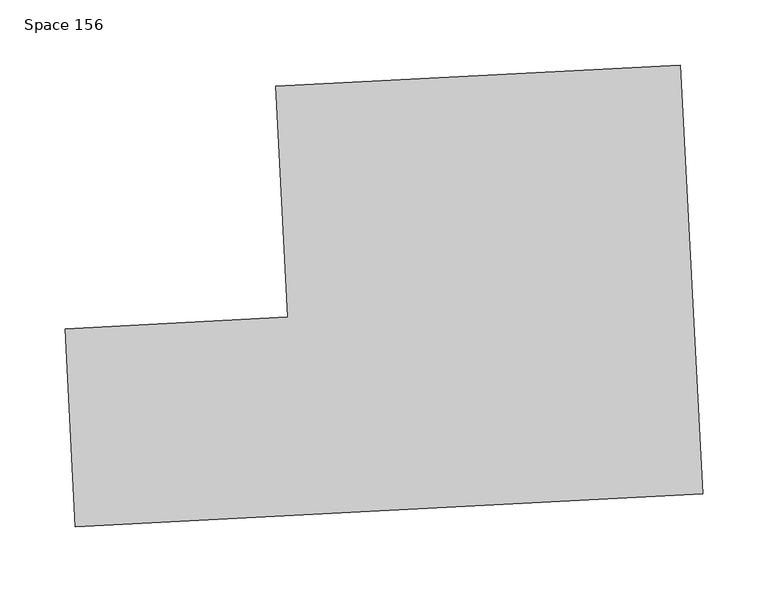
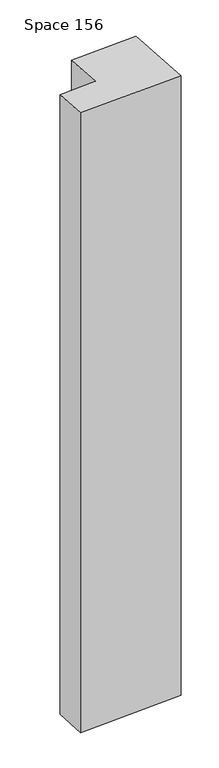
"""IFC4 building model written with IfcOpenShell, lengths in millimetres: proxy geometry, Space 156."""

from ifc_helpers import new_model, si_unit, frame, origin, place, context, project, spatial, polyline, outline, extrude, source, transform, mapped, element, save


def space_156_bf02bf6d(model_context):
    return source(origin(), model_context, "Body", "SweptSolid", [
        extrude(outline(polyline([(6675.6990245, -35006.9418992), (6667.7230248, -34854.7507581), (6838.9380585, -34845.7777585), (6829.6327255, -34668.2214272), (7140.3563053, -34651.9370944), (7157.637638, -34981.6845668), (6675.6990245, -35006.9418992)])), frame((0.0, 0.0, 3810.0), z_axis=(0.0, 0.0, 1.0), x_axis=(1.0, 0.0, 0.0)), (0.0, 0.0, 1.0), 3048.0),
    ])


if __name__ == "__main__":
    model = new_model("IFC4")
    model_context = context("Model", 3, world=origin())
    ifc_project = project(units=[si_unit("LENGTHUNIT", "METRE", prefix="MILLI")], contexts=[model_context])
    site = spatial("IfcSite", under=ifc_project)
    building = spatial("IfcBuilding", under=site)
    placement = place(None, origin())
    space_156_shape = space_156_bf02bf6d(model_context)
    element("IfcBuildingElementProxy", 1, Name="Space 156", ObjectType="Space 156", at=placement, inside=building, context=model_context, shape_type="MappedRepresentation", body=[
        mapped(space_156_shape, transform((0.0, 0.0, 0.0), x_axis=(1.0, 0.0, 0.0), y_axis=(0.0, 1.0, 0.0), z_axis=(0.0, 0.0, 1.0))),
    ])
    save(model, "model.ifc")

# Revit data of these elements
# Element 1 (IfcBuildingElementProxy, "Space 156")
#   Materials on its faces: "Render Material 255-255-255"
# Materials
#   "Render Material 255-255-255": class "Unassigned", colour RGB 255 255 255, transparency 0
